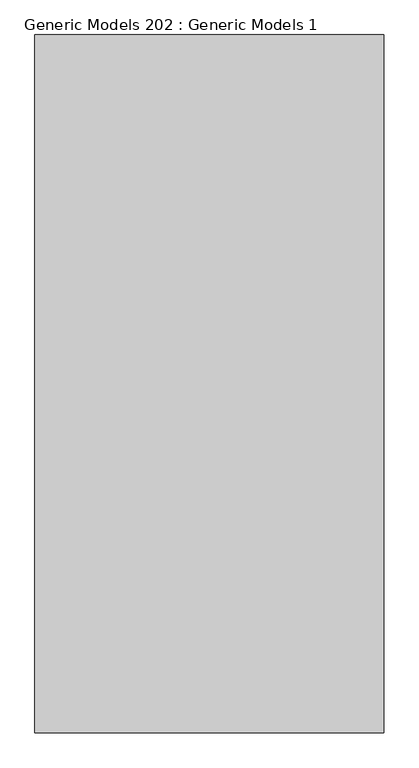
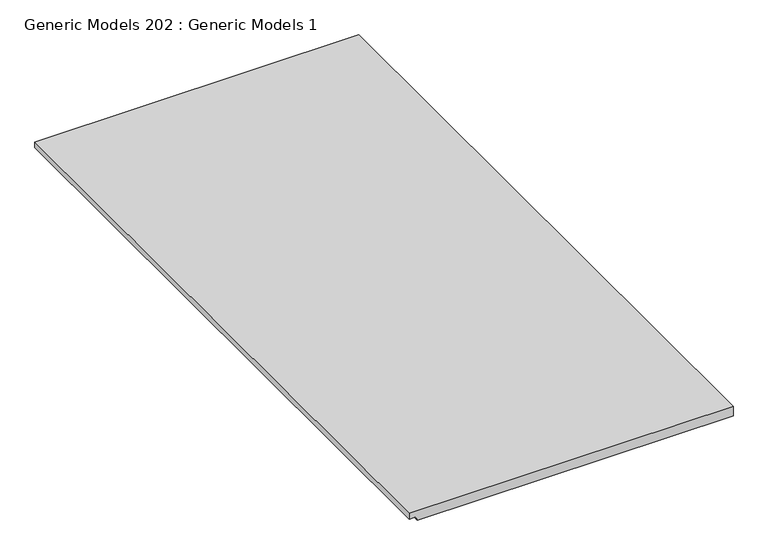
"""IFC4 building model written with IfcOpenShell, lengths in millimetres: proxy geometry, Generic Models 202 : Generic Models 1."""

from ifc_helpers import new_model, si_unit, frame, origin, place, context, project, spatial, polyline, outline, extrude, source, transform, mapped, element, save


def generic_models_202_generic_models_1_0ad20a8b(model_context):
    return source(origin(), model_context, "Body", "SweptSolid", [
        extrude(outline(polyline([(2253.330428, 49813.3451407), (2242.217928, 49813.3451407), (2242.217928, 49826.0451407), (2234.280428, 49828.9341545), (2234.280428, 50422.9451407), (2253.330428, 50422.9451407), (2253.330428, 49813.3451407)])), frame((0.0, 0.0, 0.0), z_axis=(0.0, 1.0, 0.0), x_axis=(0.0, 0.0, 1.0)), (0.0, 0.0, 1.0), 1219.2),
    ])


if __name__ == "__main__":
    model = new_model("IFC4")
    model_context = context("Model", 3, world=origin())
    ifc_project = project(units=[si_unit("LENGTHUNIT", "METRE", prefix="MILLI")], contexts=[model_context])
    site = spatial("IfcSite", under=ifc_project)
    building = spatial("IfcBuilding", under=site)
    placement = place(None, origin())
    generic_models_202_generic_models_1_shape = generic_models_202_generic_models_1_0ad20a8b(model_context)
    element("IfcBuildingElementProxy", 1, Name="Generic Models 202 : Generic Models 1", ObjectType="Generic Models 202 : Generic Models 1", at=placement, inside=building, context=model_context, shape_type="MappedRepresentation", body=[
        mapped(generic_models_202_generic_models_1_shape, transform((0.0, 0.0, 0.0), x_axis=(1.0, 0.0, 0.0), y_axis=(0.0, 1.0, 0.0), z_axis=(0.0, 0.0, 1.0))),
    ])
    save(model, "model.ifc")

# Revit data of these elements
# Element 1 (IfcBuildingElementProxy, "Generic Models 202 : Generic Models 1")
#   Materials on its faces: "CEILING AS SCHEDULED"
# Materials
#   "CEILING AS SCHEDULED": class "Generic", colour RGB 255 255 255, transparency 0, Cost = 0
